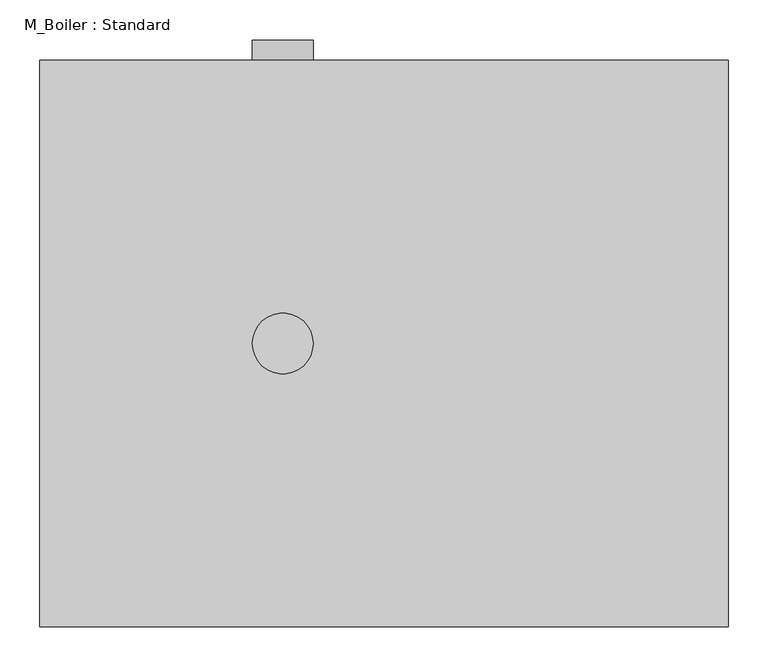
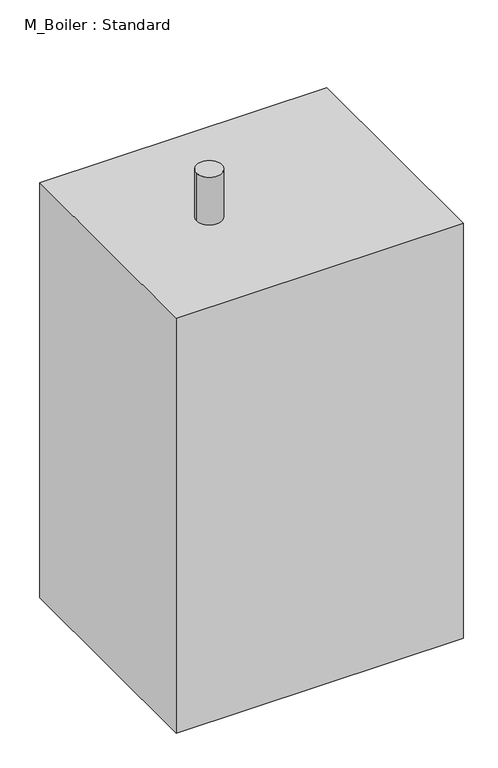
"""IFC4 building model written with IfcOpenShell, lengths in millimetres: proxy geometry, M_Boiler : Standard."""

from ifc_helpers import new_model, si_unit, point, frame, frame_2d, origin, origin_with_axes, place, context, project, spatial, polyline, circle_curve, trimmed, segment, composite_curve, outline, extrude, source, transform, mapped, element, save


def m_boiler_standard_843959aa(model_context):
    return source(origin(), model_context, "Body", "SweptSolid", [
        extrude(outline(polyline([(863.6, 0.0), (0.0, 0.0), (0.0, 711.2), (863.6, 711.2), (863.6, 0.0)])), origin_with_axes(), (0.0, 0.0, 1.0), 1320.8),
        extrude(outline(composite_curve([segment(trimmed(circle_curve(frame_2d((304.8, 355.6)), 38.1), [point((266.7, 355.6))], [point((342.9, 355.6))], False, "CARTESIAN"), True, "CONTINUOUS"), segment(trimmed(circle_curve(frame_2d((304.8, 355.6)), 38.1), [point((342.9, 355.6))], [point((266.7, 355.6))], False, "CARTESIAN"), True, "CONTINUOUS")], self_intersect=False)), frame((0.0, 0.0, 1320.8), z_axis=(0.0, 0.0, 1.0), x_axis=(1.0, 0.0, 0.0)), (0.0, 0.0, 1.0), 152.4),
        extrude(outline(composite_curve([segment(trimmed(circle_curve(frame_2d((254.0, 304.8)), 38.1), [point((254.0, 342.9))], [point((254.0, 266.7))], False, "CARTESIAN"), True, "CONTINUOUS"), segment(trimmed(circle_curve(frame_2d((254.0, 304.8)), 38.1), [point((254.0, 266.7))], [point((254.0, 342.9))], False, "CARTESIAN"), True, "CONTINUOUS")], self_intersect=False)), frame((0.0, 711.2, 0.0), z_axis=(0.0, 1.0, 0.0), x_axis=(0.0, 0.0, 1.0)), (0.0, 0.0, 1.0), 25.4),
    ])


if __name__ == "__main__":
    model = new_model("IFC4")
    model_context = context("Model", 3, world=origin())
    ifc_project = project(units=[si_unit("LENGTHUNIT", "METRE", prefix="MILLI")], contexts=[model_context])
    site = spatial("IfcSite", under=ifc_project)
    building = spatial("IfcBuilding", under=site)
    placement = place(None, origin())
    m_boiler_standard_shape = m_boiler_standard_843959aa(model_context)
    element("IfcBuildingElementProxy", 1, Name="M_Boiler : Standard", ObjectType="M_Boiler : Standard", at=placement, inside=building, context=model_context, shape_type="MappedRepresentation", body=[
        mapped(m_boiler_standard_shape, transform((0.0, 0.0, 0.0), x_axis=(1.0, 0.0, 0.0), y_axis=(0.0, 1.0, 0.0), z_axis=(0.0, 0.0, 1.0))),
    ])
    save(model, "model.ifc")

# Revit data of these elements
# Project information
#   Название организации = "Organization Name"
#   Описание организации = "Organization Description"
#   Наименование здания = "Building Name"
#   Дата утверждения проекта = "Issue Date"
#   Статус проекта = "Project Status"
#   Заказчик = "Client Name"
#   Адрес проекта = "Enter address here\nAddress Line 2"
#   Наименование проекта = "Project Name"
#   Номер проекта = "Project Number"
# Type "M_Boiler : Standard"
#   Pressure Drop [instance default] = 11700.0 Pa
#   Max Flow [instance default] = 14.5 L/s
#   Connector = 40 mm
#   Default Elevation = 0
